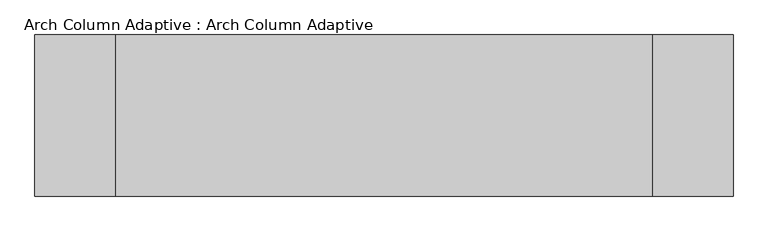
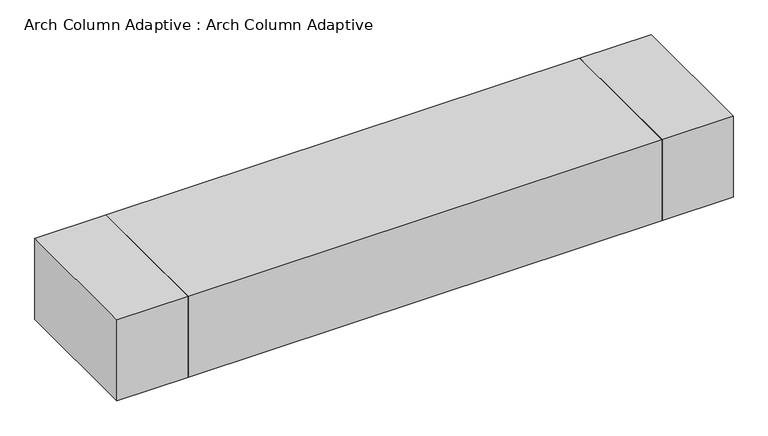
"""IFC4 building model written with IfcOpenShell, lengths in millimetres: proxy geometry, Arch Column Adaptive : Arch Column Adaptive."""

import ifcopenshell
import ifcopenshell.guid

model = None  # the IFC model being written
_history = None  # IfcOwnerHistory: only IFC2X3 demands one
_inside = {}  # id of a spatial element -> (the spatial element, [elements in it])
_under = {}  # id of a project, library or spatial element -> (it, [spatial elements below it])
_declared = {}  # id of a project -> (the project, [libraries it declares])
_typed = {}  # id of a type object -> (the type object, [elements of that type])
_made_of = {}  # id of a material, layer set ... -> (it, [elements and type objects made of it])


def new_model(schema):
    """Start an empty IFC model of exactly this schema.

    Asked for "IFC4X3", IfcOpenShell would pick the latest addendum, in which some entities
    have other attributes; the version numbers below select the first issue.
    IFC2X3 requires an IfcOwnerHistory on every rooted entity: one is made here for all.
    """
    global model, _history
    if schema == "IFC4X3":
        model = ifcopenshell.file(schema_version=(4, 3, 0, 0))
    else:
        model = ifcopenshell.file(schema=schema)
    _inside.clear()
    _under.clear()
    _declared.clear()
    _typed.clear()
    _made_of.clear()
    _history = None
    if model.schema == "IFC2X3":
        org = make("IfcOrganization", Name="unknown")
        user = make(
            "IfcPersonAndOrganization",
            ThePerson=make("IfcPerson", FamilyName="unknown"),
            TheOrganization=org,
        )
        app = make(
            "IfcApplication",
            ApplicationDeveloper=org,
            Version="unknown",
            ApplicationFullName="unknown",
            ApplicationIdentifier="unknown",
        )
        _history = make(
            "IfcOwnerHistory",
            OwningUser=user,
            OwningApplication=app,
            ChangeAction="ADDED",
            CreationDate=0,
        )
    return model


def make(cls, **values):
    """One entity of the class cls with the attributes given. An attribute that is None is left unset."""
    return model.create_entity(
        cls, **{name: value for name, value in values.items() if value is not None}
    )


def rooted(cls, **values):
    """An entity with a GlobalId (a new one), such as an element, a storey or a relation."""
    return make(cls, GlobalId=ifcopenshell.guid.new(), OwnerHistory=_history, **values)


def si_unit(unit_type, name, prefix=None):
    """IfcSIUnit, for example si_unit("LENGTHUNIT", "METRE", prefix="MILLI")."""
    return make("IfcSIUnit", UnitType=unit_type, Prefix=prefix, Name=name)


def assignment(units):
    """IfcUnitAssignment: the units of a project."""
    return None if units is None else make("IfcUnitAssignment", Units=units)


def point(xyz):
    """IfcCartesianPoint."""
    return None if xyz is None else make("IfcCartesianPoint", Coordinates=xyz)


def direction(xyz):
    """IfcDirection."""
    return None if xyz is None else make("IfcDirection", DirectionRatios=xyz)


def frame(location, z_axis=None, x_axis=None):
    """IfcAxis2Placement3D, a coordinate frame: its origin and axes. An axis left out is left unset."""
    return make(
        "IfcAxis2Placement3D",
        Location=point(location),
        Axis=direction(z_axis),
        RefDirection=direction(x_axis),
    )


def origin():
    """The frame at (0, 0, 0) with its axes left unset."""
    return frame((0.0, 0.0, 0.0))


def place(relative_to, where):
    """IfcLocalPlacement: puts the frame where relative to a parent placement (None: the world)."""
    return make(
        "IfcLocalPlacement", PlacementRelTo=relative_to, RelativePlacement=where
    )


def context(
    kind, dimensions, precision=None, world=None, true_north=None, identifier=None
):
    """IfcGeometricRepresentationContext, for example the 3D "Model" context."""
    return make(
        "IfcGeometricRepresentationContext",
        ContextIdentifier=identifier,
        ContextType=kind,
        CoordinateSpaceDimension=dimensions,
        Precision=precision,
        WorldCoordinateSystem=world,
        TrueNorth=true_north,
    )


def project(units=None, contexts=None):
    """IfcProject with its units and contexts."""
    return rooted(
        "IfcProject",
        Name="project",
        RepresentationContexts=contexts,
        UnitsInContext=assignment(units),
    )


def spatial(cls, under=None, at=None, **own):
    """A site, building, storey or space (cls), placed at a placement, below another one or the project."""
    s = rooted(cls, ObjectPlacement=at, **own)
    if under is not None:
        _under.setdefault(under.id(), (under, []))[1].append(s)
    return s


def polyline(points):
    """IfcPolyline through the points."""
    return make("IfcPolyline", Points=[point(p) for p in points])


def outline(outer, holes=None, kind="AREA"):
    """IfcArbitraryClosedProfileDef: a profile drawn as a closed curve; with holes, ...WithVoids."""
    if holes is None:
        return make("IfcArbitraryClosedProfileDef", ProfileType=kind, OuterCurve=outer)
    return make(
        "IfcArbitraryProfileDefWithVoids",
        ProfileType=kind,
        OuterCurve=outer,
        InnerCurves=holes,
    )


def extrude(swept, where, along, depth):
    """IfcExtrudedAreaSolid: the profile swept, set in the frame where, extruded along a direction by depth."""
    return make(
        "IfcExtrudedAreaSolid",
        SweptArea=swept,
        Position=where,
        ExtrudedDirection=direction(along),
        Depth=depth,
    )


def shape(context_of_items, identifier, shape_type, items):
    """IfcShapeRepresentation: the items that make up one representation, for example the "Body"."""
    return make(
        "IfcShapeRepresentation",
        ContextOfItems=context_of_items,
        RepresentationIdentifier=identifier,
        RepresentationType=shape_type,
        Items=items,
    )


def source(mapping_origin, context_of_items, identifier, shape_type, items):
    """IfcRepresentationMap: a shape defined once, which mapped items show again and again."""
    return make(
        "IfcRepresentationMap",
        MappingOrigin=mapping_origin,
        MappedRepresentation=shape(context_of_items, identifier, shape_type, items),
    )


def transform(
    local_origin,
    x_axis=None,
    y_axis=None,
    z_axis=None,
    scale=None,
    scale2=None,
    scale3=None,
    uniform=True,
):
    """IfcCartesianTransformationOperator3D, or its non-uniform kind. x_axis, y_axis, z_axis: its Axis1, 2, 3."""
    if uniform:
        return make(
            "IfcCartesianTransformationOperator3D",
            Axis1=direction(x_axis),
            Axis2=direction(y_axis),
            LocalOrigin=point(local_origin),
            Scale=scale,
            Axis3=direction(z_axis),
        )
    return make(
        "IfcCartesianTransformationOperator3DnonUniform",
        Axis1=direction(x_axis),
        Axis2=direction(y_axis),
        LocalOrigin=point(local_origin),
        Scale=scale,
        Axis3=direction(z_axis),
        Scale2=scale2,
        Scale3=scale3,
    )


def mapped(mapping_source, mapping_target):
    """IfcMappedItem: shows the shape of a source again, moved by a transform."""
    return make(
        "IfcMappedItem", MappingSource=mapping_source, MappingTarget=mapping_target
    )


def made_of(thing, what):
    """Note that an element or type object is made of a material, layer set ...; save() writes the relation."""
    if what is not None:
        _made_of.setdefault(what.id(), (what, []))[1].append(thing)
    return thing


def element(
    cls,
    number,
    at=None,
    inside=None,
    cuts=None,
    type_object=None,
    material=None,
    context=None,
    identifier="Body",
    shape_type=None,
    held_by="IfcProductDefinitionShape",
    body=None,
    shapes=None,
    **own,
):
    """One element of the class cls, such as IfcWall. Its Tag is "e" and its number.

    at: its placement. inside: the storey or other place that contains it. cuts: it is an
    opening in that element (IfcRelVoidsElement). A single representation is given by context,
    identifier, shape_type and body (its items); several are given by shapes. held_by: the class
    of the entity that holds the representations. save() writes the other relations.
    """
    e = rooted(cls, Tag="e%d" % number, ObjectPlacement=at, **own)
    if body is not None:
        shapes = [shape(context, identifier, shape_type, body)]
    if shapes is not None:
        e.Representation = make(held_by, Representations=shapes)
    if inside is not None:
        _inside.setdefault(inside.id(), (inside, []))[1].append(e)
    if cuts is not None:
        rooted(
            "IfcRelVoidsElement", RelatingBuildingElement=cuts, RelatedOpeningElement=e
        )
    if type_object is not None:
        _typed.setdefault(type_object.id(), (type_object, []))[1].append(e)
    return made_of(e, material)


def aggregate(whole, parts):
    """IfcRelAggregates: a whole, such as a stair, and the parts it consists of."""
    return rooted("IfcRelAggregates", RelatingObject=whole, RelatedObjects=parts)


def save(model, path):
    """Write the relations noted so far, then the file.

    IfcRelAggregates (storeys below a building ...), IfcRelContainedInSpatialStructure (elements
    in a storey), IfcRelDefinesByType, IfcRelAssociatesMaterial and IfcRelDeclares: one each for
    every whole, place, type object, material and project.
    """
    for whole, parts in _under.values():
        aggregate(whole, parts)
    for where, things in _inside.values():
        rooted(
            "IfcRelContainedInSpatialStructure",
            RelatedElements=things,
            RelatingStructure=where,
        )
    for kind, things in _typed.values():
        rooted("IfcRelDefinesByType", RelatedObjects=things, RelatingType=kind)
    for what, things in _made_of.values():
        rooted("IfcRelAssociatesMaterial", RelatedObjects=things, RelatingMaterial=what)
    for by, libraries in _declared.values():
        rooted("IfcRelDeclares", RelatingContext=by, RelatedDefinitions=libraries)
    model.write(path)


def arch_column_adaptive_arch_column_adaptive_582f5647(model_context):
    return source(origin(), model_context, "Body", "SweptSolid", [
        extrude(outline(polyline([(5000.0, -1500.0), (5000.0, 1500.0), (6500.0, 1500.0), (6500.0, -1500.0), (5000.0, -1500.0)])), frame((0.0, 0.0, 43700.0), z_axis=(0.0, 0.0, 1.0), x_axis=(1.0, 0.0, 0.0)), (0.0, 0.0, 1.0), 1800.0),
        extrude(outline(polyline([(-5000.0, 1500.0), (-5000.0, -1500.0), (-6500.0, -1500.0), (-6500.0, 1500.0), (-5000.0, 1500.0)])), frame((0.0, 0.0, 43700.0), z_axis=(0.0, 0.0, 1.0), x_axis=(1.0, 0.0, 0.0)), (0.0, 0.0, 1.0), 1800.0),
        extrude(outline(polyline([(-5000.0, -1500.0), (-5000.0, 1500.0), (5000.0, 1500.0), (5000.0, -1500.0), (-5000.0, -1500.0)])), frame((0.0, 0.0, 43700.0), z_axis=(0.0, 0.0, 1.0), x_axis=(1.0, 0.0, 0.0)), (0.0, 0.0, 1.0), 1800.0),
    ])


if __name__ == "__main__":
    model = new_model("IFC4")
    model_context = context("Model", 3, world=origin())
    ifc_project = project(units=[si_unit("LENGTHUNIT", "METRE", prefix="MILLI")], contexts=[model_context])
    site = spatial("IfcSite", under=ifc_project)
    building = spatial("IfcBuilding", under=site)
    placement = place(None, origin())
    arch_column_adaptive_arch_column_adaptive_shape = arch_column_adaptive_arch_column_adaptive_582f5647(model_context)
    element("IfcBuildingElementProxy", 1, Name="Arch Column Adaptive : Arch Column Adaptive", ObjectType="Arch Column Adaptive : Arch Column Adaptive", at=placement, inside=building, context=model_context, shape_type="MappedRepresentation", body=[
        mapped(arch_column_adaptive_arch_column_adaptive_shape, transform((0.0, 0.0, 0.0), x_axis=(1.0, 0.0, 0.0), y_axis=(0.0, 1.0, 0.0), z_axis=(0.0, 0.0, 1.0))),
    ])
    save(model, "model.ifc")

# Revit data of these elements
# Type "Arch Column Adaptive : Arch Column Adaptive"
#   Top Width = 3000 mm
#   Length [instance default] = 21000 mm
#   Height [instance default] = 50000 mm
#   Default Elevation = 0
# Element 1 (IfcBuildingElementProxy, "Arch Column Adaptive : Arch Column Adaptive")
#   Height = 43700 mm
